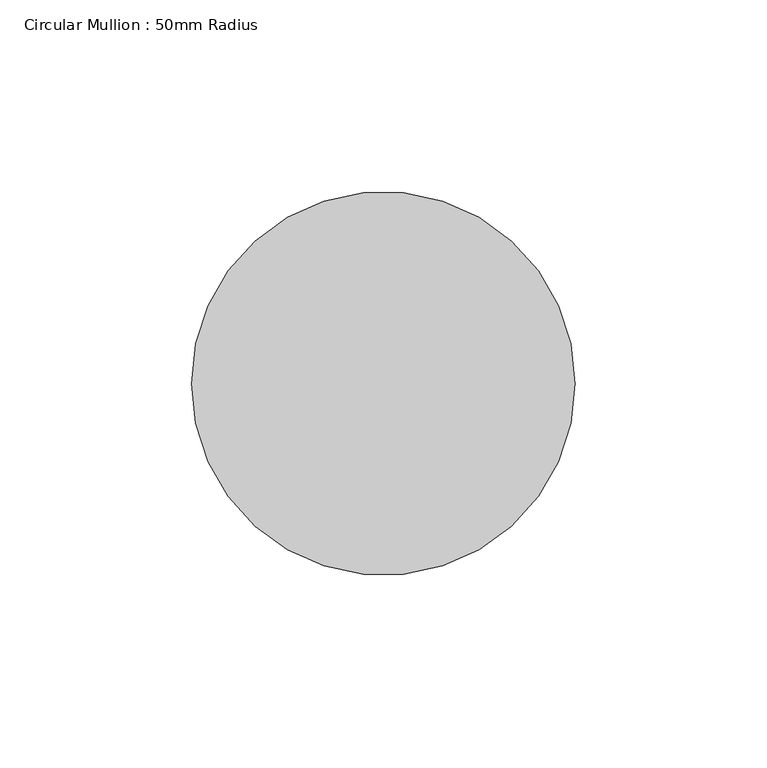
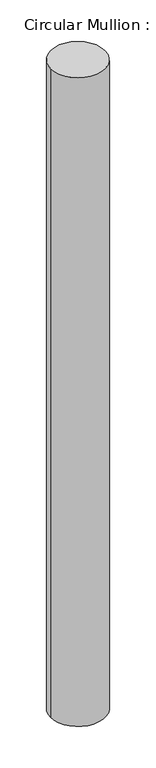
"""IFC4 building model written with IfcOpenShell, lengths in millimetres: member geometry, Circular Mullion : 50mm Radius."""

from ifc_helpers import new_model, si_unit, point, frame, origin, origin_2d, place, context, project, spatial, circle_curve, trimmed, segment, composite_curve, outline, extrude, source, transform, mapped, element, save


def circular_mullion_50mm_radius_008be280(model_context):
    return source(origin(), model_context, "Body", "SweptSolid", [
        extrude(outline(composite_curve([segment(trimmed(circle_curve(origin_2d(), 50.0), [point((50.0, 0.0))], [point((-50.0, 0.0))], False, "CARTESIAN"), True, "CONTINUOUS"), segment(trimmed(circle_curve(origin_2d(), 50.0), [point((-50.0, 0.0))], [point((50.0, 0.0))], False, "CARTESIAN"), True, "CONTINUOUS")], self_intersect=False)), frame((0.0, 0.0, -1254.4478539), z_axis=(0.0, 0.0, 1.0), x_axis=(1.0, 0.0, 0.0)), (0.0, 0.0, 1.0), 1254.4478539),
    ])


if __name__ == "__main__":
    model = new_model("IFC4")
    model_context = context("Model", 3, world=origin())
    ifc_project = project(units=[si_unit("LENGTHUNIT", "METRE", prefix="MILLI")], contexts=[model_context])
    site = spatial("IfcSite", under=ifc_project)
    building = spatial("IfcBuilding", under=site)
    placement = place(None, origin())
    circular_mullion_50mm_radius_shape = circular_mullion_50mm_radius_008be280(model_context)
    element("IfcMember", 1, ObjectType="Circular Mullion : 50mm Radius", at=placement, inside=building, context=model_context, shape_type="MappedRepresentation", body=[
        mapped(circular_mullion_50mm_radius_shape, transform((0.0, 0.0, 0.0), x_axis=(1.0, 0.0, 0.0), y_axis=(0.0, 1.0, 0.0), z_axis=(0.0, 0.0, 1.0))),
    ])
    save(model, "model.ifc")

# Revit data of these elements
# Project information
#   Project Issue Date = "Issue Date"
#   Project Status = "Project Status"
#   Client Name = "Owner"
#   Project Address = "Enter address here"
#   Project Name = "Project Name"
#   Project Number = "0001"
# Type "Circular Mullion : 50mm Radius"
#   built-in parameter 1007350 = 0.164042 (stored number, unit not read)
# Element 1 (IfcMember, "Circular Mullion : 50mm Radius")
#   Materials on its faces: "Aluminium"
# Materials
#   "Aluminium": class "Metal", colour RGB 247 247 247, transparency 0, Description = "Aluminium 6061", Cost = 0
